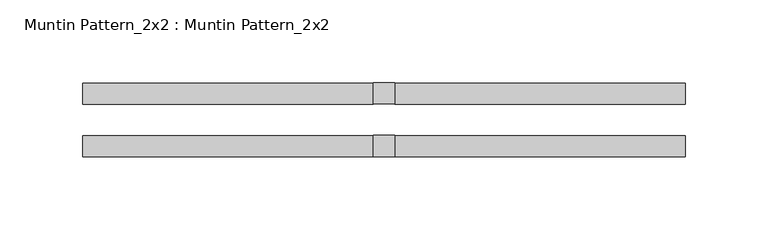
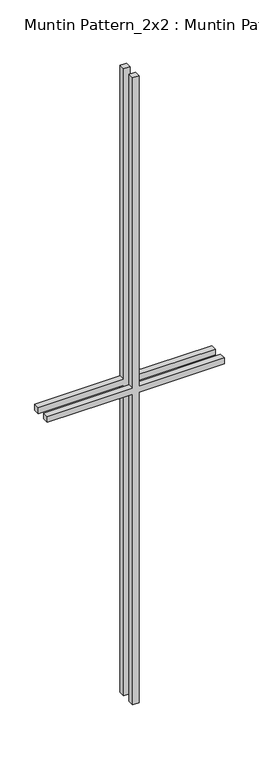
"""IFC4 building model written with IfcOpenShell, lengths in millimetres: proxy geometry, Muntin Pattern_2x2 : Muntin Pattern_2x2."""

from ifc_helpers import new_model, si_unit, frame, origin, place, context, project, spatial, polyline, outline, extrude, source, transform, mapped, element, save


def muntin_pattern_2x2_muntin_pattern_2x2_cbb9fd28(model_context):
    return source(origin(), model_context, "Body", "SweptSolid", [
        extrude(outline(polyline([(686.5, -6.35), (686.5, -181.7375), (673.8, -181.7375), (673.8, -6.35), (0.0, -6.35), (0.0, 6.35), (673.8, 6.35), (673.8, 181.7375), (686.5, 181.7375), (686.5, 6.35), (1360.3, 6.35), (1360.3, -6.35), (686.5, -6.35)])), frame((0.0, 9.525, 0.0), z_axis=(0.0, 1.0, 0.0), x_axis=(0.0, 0.0, 1.0)), (0.0, 0.0, 1.0), 12.7),
        extrude(outline(polyline([(686.5, -6.35), (686.5, -181.7375), (673.8, -181.7375), (673.8, -6.35), (0.0, -6.35), (0.0, 6.35), (673.8, 6.35), (673.8, 181.7375), (686.5, 181.7375), (686.5, 6.35), (1360.3, 6.35), (1360.3, -6.35), (686.5, -6.35)])), frame((0.0, -22.225, 0.0), z_axis=(0.0, 1.0, 0.0), x_axis=(0.0, 0.0, 1.0)), (0.0, 0.0, 1.0), 12.7),
    ])


if __name__ == "__main__":
    model = new_model("IFC4")
    model_context = context("Model", 3, world=origin())
    ifc_project = project(units=[si_unit("LENGTHUNIT", "METRE", prefix="MILLI")], contexts=[model_context])
    site = spatial("IfcSite", under=ifc_project)
    building = spatial("IfcBuilding", under=site)
    placement = place(None, origin())
    muntin_pattern_2x2_muntin_pattern_2x2_shape = muntin_pattern_2x2_muntin_pattern_2x2_cbb9fd28(model_context)
    element("IfcBuildingElementProxy", 1, Name="Muntin Pattern_2x2 : Muntin Pattern_2x2", ObjectType="Muntin Pattern_2x2 : Muntin Pattern_2x2", at=placement, inside=building, context=model_context, shape_type="MappedRepresentation", body=[
        mapped(muntin_pattern_2x2_muntin_pattern_2x2_shape, transform((0.0, 0.0, 0.0), x_axis=(1.0, 0.0, 0.0), y_axis=(0.0, 1.0, 0.0), z_axis=(0.0, 0.0, 1.0))),
    ])
    save(model, "model.ifc")

# Revit data of these elements
# Type "Muntin Pattern_2x2 : Muntin Pattern_2x2"
#   Width [instance default] = 121.92 cm
#   Thickness = 1.27 cm
#   Height [instance default] = 121.92 cm
#   Distance = 1.905 cm
#   Interior Material [instance default] = none
#   Exterior Material [instance default] = none
# Element 1 (IfcBuildingElementProxy, "Muntin Pattern_2x2 : Muntin Pattern_2x2")
#   Width = 36.3475 cm
#   Height = 136.03 cm
#   Interior Material = Wood - Stained
#   Exterior Material = Clad - White
#   Materials on its faces: "Clad - White", "Wood - Stained"
# Materials
#   "Clad - White": class "Wood", colour RGB 242 242 238, transparency 0, Cost = 0
#   "Wood - Stained": class "Wood", colour RGB 224 178 126, transparency 0, Cost = 0
